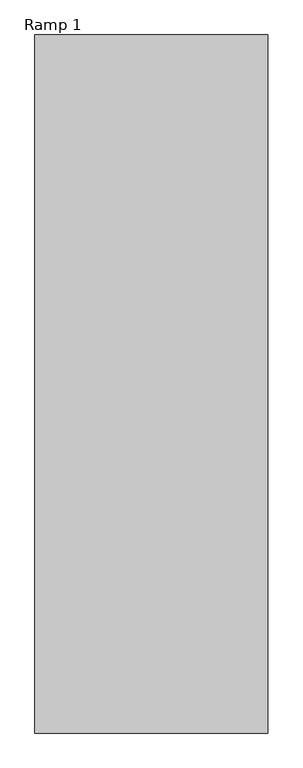
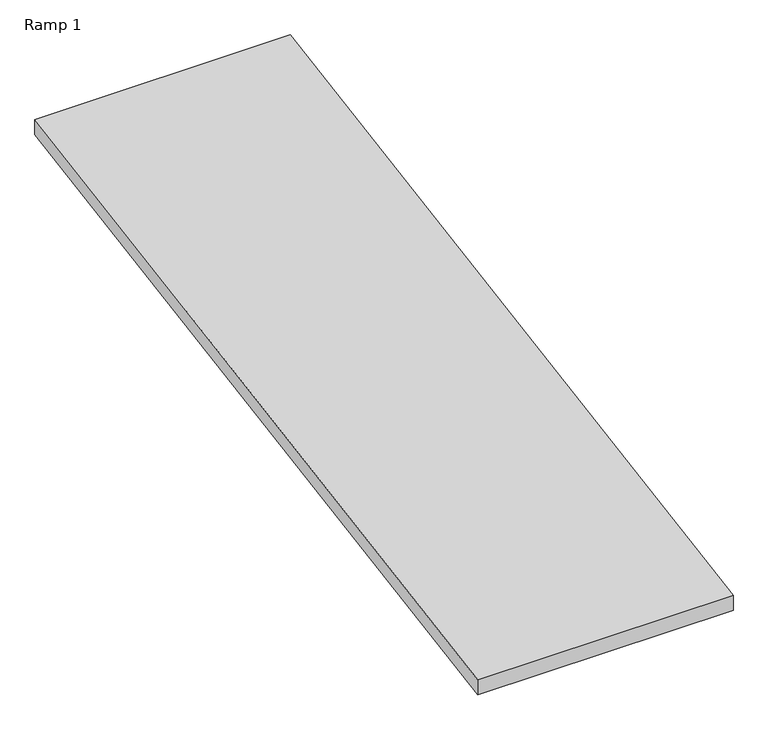
"""IFC4 building model written with IfcOpenShell, lengths in millimetres: ramp geometry, Ramp 1."""

import ifcopenshell
import ifcopenshell.guid

model = None  # the IFC model being written
_history = None  # IfcOwnerHistory: only IFC2X3 demands one
_inside = {}  # id of a spatial element -> (the spatial element, [elements in it])
_under = {}  # id of a project, library or spatial element -> (it, [spatial elements below it])
_declared = {}  # id of a project -> (the project, [libraries it declares])
_typed = {}  # id of a type object -> (the type object, [elements of that type])
_made_of = {}  # id of a material, layer set ... -> (it, [elements and type objects made of it])


def new_model(schema):
    """Start an empty IFC model of exactly this schema.

    Asked for "IFC4X3", IfcOpenShell would pick the latest addendum, in which some entities
    have other attributes; the version numbers below select the first issue.
    IFC2X3 requires an IfcOwnerHistory on every rooted entity: one is made here for all.
    """
    global model, _history
    if schema == "IFC4X3":
        model = ifcopenshell.file(schema_version=(4, 3, 0, 0))
    else:
        model = ifcopenshell.file(schema=schema)
    _inside.clear()
    _under.clear()
    _declared.clear()
    _typed.clear()
    _made_of.clear()
    _history = None
    if model.schema == "IFC2X3":
        org = make("IfcOrganization", Name="unknown")
        user = make(
            "IfcPersonAndOrganization",
            ThePerson=make("IfcPerson", FamilyName="unknown"),
            TheOrganization=org,
        )
        app = make(
            "IfcApplication",
            ApplicationDeveloper=org,
            Version="unknown",
            ApplicationFullName="unknown",
            ApplicationIdentifier="unknown",
        )
        _history = make(
            "IfcOwnerHistory",
            OwningUser=user,
            OwningApplication=app,
            ChangeAction="ADDED",
            CreationDate=0,
        )
    return model


def make(cls, **values):
    """One entity of the class cls with the attributes given. An attribute that is None is left unset."""
    return model.create_entity(
        cls, **{name: value for name, value in values.items() if value is not None}
    )


def rooted(cls, **values):
    """An entity with a GlobalId (a new one), such as an element, a storey or a relation."""
    return make(cls, GlobalId=ifcopenshell.guid.new(), OwnerHistory=_history, **values)


def si_unit(unit_type, name, prefix=None):
    """IfcSIUnit, for example si_unit("LENGTHUNIT", "METRE", prefix="MILLI")."""
    return make("IfcSIUnit", UnitType=unit_type, Prefix=prefix, Name=name)


def assignment(units):
    """IfcUnitAssignment: the units of a project."""
    return None if units is None else make("IfcUnitAssignment", Units=units)


def point(xyz):
    """IfcCartesianPoint."""
    return None if xyz is None else make("IfcCartesianPoint", Coordinates=xyz)


def direction(xyz):
    """IfcDirection."""
    return None if xyz is None else make("IfcDirection", DirectionRatios=xyz)


def frame(location, z_axis=None, x_axis=None):
    """IfcAxis2Placement3D, a coordinate frame: its origin and axes. An axis left out is left unset."""
    return make(
        "IfcAxis2Placement3D",
        Location=point(location),
        Axis=direction(z_axis),
        RefDirection=direction(x_axis),
    )


def origin():
    """The frame at (0, 0, 0) with its axes left unset."""
    return frame((0.0, 0.0, 0.0))


def place(relative_to, where):
    """IfcLocalPlacement: puts the frame where relative to a parent placement (None: the world)."""
    return make(
        "IfcLocalPlacement", PlacementRelTo=relative_to, RelativePlacement=where
    )


def context(
    kind, dimensions, precision=None, world=None, true_north=None, identifier=None
):
    """IfcGeometricRepresentationContext, for example the 3D "Model" context."""
    return make(
        "IfcGeometricRepresentationContext",
        ContextIdentifier=identifier,
        ContextType=kind,
        CoordinateSpaceDimension=dimensions,
        Precision=precision,
        WorldCoordinateSystem=world,
        TrueNorth=true_north,
    )


def project(units=None, contexts=None):
    """IfcProject with its units and contexts."""
    return rooted(
        "IfcProject",
        Name="project",
        RepresentationContexts=contexts,
        UnitsInContext=assignment(units),
    )


def spatial(cls, under=None, at=None, **own):
    """A site, building, storey or space (cls), placed at a placement, below another one or the project."""
    s = rooted(cls, ObjectPlacement=at, **own)
    if under is not None:
        _under.setdefault(under.id(), (under, []))[1].append(s)
    return s


def polyline(points):
    """IfcPolyline through the points."""
    return make("IfcPolyline", Points=[point(p) for p in points])


def outline(outer, holes=None, kind="AREA"):
    """IfcArbitraryClosedProfileDef: a profile drawn as a closed curve; with holes, ...WithVoids."""
    if holes is None:
        return make("IfcArbitraryClosedProfileDef", ProfileType=kind, OuterCurve=outer)
    return make(
        "IfcArbitraryProfileDefWithVoids",
        ProfileType=kind,
        OuterCurve=outer,
        InnerCurves=holes,
    )


def extrude(swept, where, along, depth):
    """IfcExtrudedAreaSolid: the profile swept, set in the frame where, extruded along a direction by depth."""
    return make(
        "IfcExtrudedAreaSolid",
        SweptArea=swept,
        Position=where,
        ExtrudedDirection=direction(along),
        Depth=depth,
    )


def shape(context_of_items, identifier, shape_type, items):
    """IfcShapeRepresentation: the items that make up one representation, for example the "Body"."""
    return make(
        "IfcShapeRepresentation",
        ContextOfItems=context_of_items,
        RepresentationIdentifier=identifier,
        RepresentationType=shape_type,
        Items=items,
    )


def source(mapping_origin, context_of_items, identifier, shape_type, items):
    """IfcRepresentationMap: a shape defined once, which mapped items show again and again."""
    return make(
        "IfcRepresentationMap",
        MappingOrigin=mapping_origin,
        MappedRepresentation=shape(context_of_items, identifier, shape_type, items),
    )


def transform(
    local_origin,
    x_axis=None,
    y_axis=None,
    z_axis=None,
    scale=None,
    scale2=None,
    scale3=None,
    uniform=True,
):
    """IfcCartesianTransformationOperator3D, or its non-uniform kind. x_axis, y_axis, z_axis: its Axis1, 2, 3."""
    if uniform:
        return make(
            "IfcCartesianTransformationOperator3D",
            Axis1=direction(x_axis),
            Axis2=direction(y_axis),
            LocalOrigin=point(local_origin),
            Scale=scale,
            Axis3=direction(z_axis),
        )
    return make(
        "IfcCartesianTransformationOperator3DnonUniform",
        Axis1=direction(x_axis),
        Axis2=direction(y_axis),
        LocalOrigin=point(local_origin),
        Scale=scale,
        Axis3=direction(z_axis),
        Scale2=scale2,
        Scale3=scale3,
    )


def mapped(mapping_source, mapping_target):
    """IfcMappedItem: shows the shape of a source again, moved by a transform."""
    return make(
        "IfcMappedItem", MappingSource=mapping_source, MappingTarget=mapping_target
    )


def made_of(thing, what):
    """Note that an element or type object is made of a material, layer set ...; save() writes the relation."""
    if what is not None:
        _made_of.setdefault(what.id(), (what, []))[1].append(thing)
    return thing


def element(
    cls,
    number,
    at=None,
    inside=None,
    cuts=None,
    type_object=None,
    material=None,
    context=None,
    identifier="Body",
    shape_type=None,
    held_by="IfcProductDefinitionShape",
    body=None,
    shapes=None,
    **own,
):
    """One element of the class cls, such as IfcWall. Its Tag is "e" and its number.

    at: its placement. inside: the storey or other place that contains it. cuts: it is an
    opening in that element (IfcRelVoidsElement). A single representation is given by context,
    identifier, shape_type and body (its items); several are given by shapes. held_by: the class
    of the entity that holds the representations. save() writes the other relations.
    """
    e = rooted(cls, Tag="e%d" % number, ObjectPlacement=at, **own)
    if body is not None:
        shapes = [shape(context, identifier, shape_type, body)]
    if shapes is not None:
        e.Representation = make(held_by, Representations=shapes)
    if inside is not None:
        _inside.setdefault(inside.id(), (inside, []))[1].append(e)
    if cuts is not None:
        rooted(
            "IfcRelVoidsElement", RelatingBuildingElement=cuts, RelatedOpeningElement=e
        )
    if type_object is not None:
        _typed.setdefault(type_object.id(), (type_object, []))[1].append(e)
    return made_of(e, material)


def aggregate(whole, parts):
    """IfcRelAggregates: a whole, such as a stair, and the parts it consists of."""
    return rooted("IfcRelAggregates", RelatingObject=whole, RelatedObjects=parts)


def save(model, path):
    """Write the relations noted so far, then the file.

    IfcRelAggregates (storeys below a building ...), IfcRelContainedInSpatialStructure (elements
    in a storey), IfcRelDefinesByType, IfcRelAssociatesMaterial and IfcRelDeclares: one each for
    every whole, place, type object, material and project.
    """
    for whole, parts in _under.values():
        aggregate(whole, parts)
    for where, things in _inside.values():
        rooted(
            "IfcRelContainedInSpatialStructure",
            RelatedElements=things,
            RelatingStructure=where,
        )
    for kind, things in _typed.values():
        rooted("IfcRelDefinesByType", RelatedObjects=things, RelatingType=kind)
    for what, things in _made_of.values():
        rooted("IfcRelAssociatesMaterial", RelatedObjects=things, RelatingMaterial=what)
    for by, libraries in _declared.values():
        rooted("IfcRelDeclares", RelatingContext=by, RelatedDefinitions=libraries)
    model.write(path)


def ramp_1_7f35b39e(model_context):
    return source(origin(), model_context, "Body", "SweptSolid", [
        extrude(outline(polyline([(-4458.4292912, 0.0), (-858.4292912, 600.0), (-858.4292912, 523.9654684), (-4458.4292912, -76.0345316), (-4458.4292912, 0.0)])), frame((-599.8488078, 0.0, 0.0), z_axis=(1.0, 0.0, 0.0), x_axis=(0.0, 1.0, 0.0)), (0.0, 0.0, 1.0), 1200.0),
    ])


if __name__ == "__main__":
    model = new_model("IFC4")
    model_context = context("Model", 3, world=origin())
    ifc_project = project(units=[si_unit("LENGTHUNIT", "METRE", prefix="MILLI")], contexts=[model_context])
    site = spatial("IfcSite", under=ifc_project)
    building = spatial("IfcBuilding", under=site)
    placement = place(None, origin())
    ramp_1_shape = ramp_1_7f35b39e(model_context)
    element("IfcRamp", 1, ObjectType="Ramp 1", at=placement, inside=building, context=model_context, shape_type="MappedRepresentation", body=[
        mapped(ramp_1_shape, transform((0.0, 0.0, 0.0), x_axis=(1.0, 0.0, 0.0), y_axis=(0.0, 1.0, 0.0), z_axis=(0.0, 0.0, 1.0))),
    ])
    save(model, "model.ifc")
